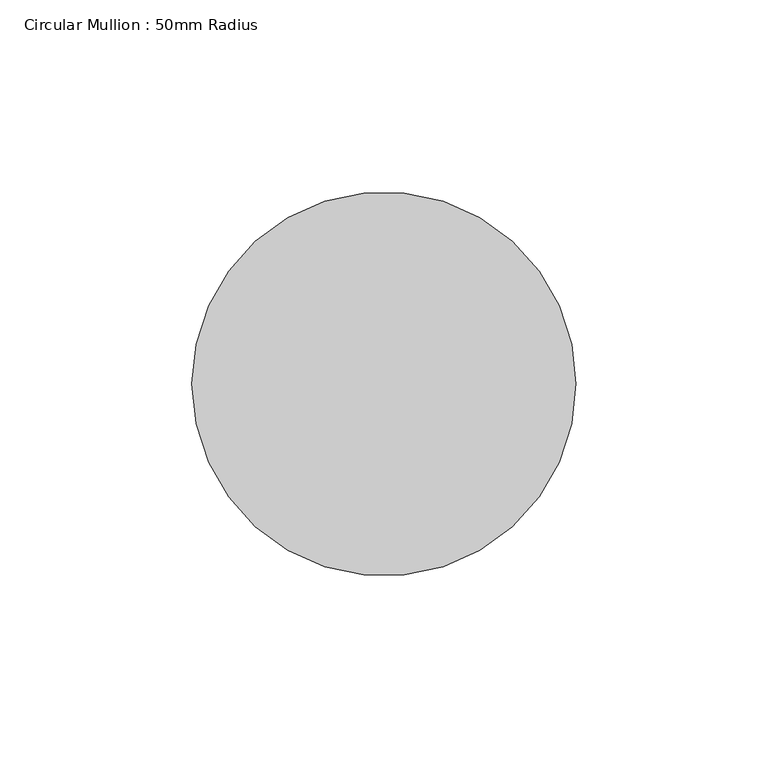
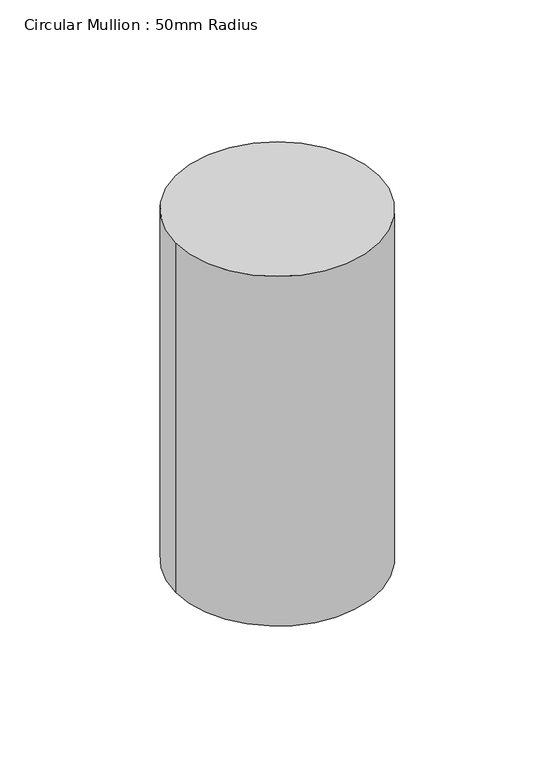
"""IFC4 building model written with IfcOpenShell, lengths in millimetres: member geometry, Circular Mullion : 50mm Radius."""

from ifc_helpers import new_model, si_unit, point, frame, origin, origin_2d, place, context, project, spatial, circle_curve, trimmed, segment, composite_curve, outline, extrude, source, transform, mapped, element, save


def circular_mullion_50mm_radius_c06fac9e(model_context):
    return source(origin(), model_context, "Body", "SweptSolid", [
        extrude(outline(composite_curve([segment(trimmed(circle_curve(origin_2d(), 50.0), [point((50.0, 0.0))], [point((-50.0, 0.0))], False, "CARTESIAN"), True, "CONTINUOUS"), segment(trimmed(circle_curve(origin_2d(), 50.0), [point((-50.0, 0.0))], [point((50.0, 0.0))], False, "CARTESIAN"), True, "CONTINUOUS")], self_intersect=False)), frame((0.0, 0.0, -181.9250532), z_axis=(0.0, 0.0, 1.0), x_axis=(1.0, 0.0, 0.0)), (0.0, 0.0, 1.0), 181.9250532),
    ])


if __name__ == "__main__":
    model = new_model("IFC4")
    model_context = context("Model", 3, world=origin())
    ifc_project = project(units=[si_unit("LENGTHUNIT", "METRE", prefix="MILLI")], contexts=[model_context])
    site = spatial("IfcSite", under=ifc_project)
    building = spatial("IfcBuilding", under=site)
    placement = place(None, origin())
    circular_mullion_50mm_radius_shape = circular_mullion_50mm_radius_c06fac9e(model_context)
    element("IfcMember", 1, ObjectType="Circular Mullion : 50mm Radius", at=placement, inside=building, context=model_context, shape_type="MappedRepresentation", body=[
        mapped(circular_mullion_50mm_radius_shape, transform((0.0, 0.0, 0.0), x_axis=(1.0, 0.0, 0.0), y_axis=(0.0, 1.0, 0.0), z_axis=(0.0, 0.0, 1.0))),
    ])
    save(model, "model.ifc")

# Revit data of these elements
# Type "Circular Mullion : 50mm Radius"
#   built-in parameter 1007350 = 0.164042 (stored number, unit not read)
# Element 1 (IfcMember, "Circular Mullion : 50mm Radius")
#   Materials on its faces: "Aluminium"
# Materials
#   "Aluminium": class "Metal", colour RGB 247 247 247, transparency 0, Description = "Aluminium 6061", Cost = 0
